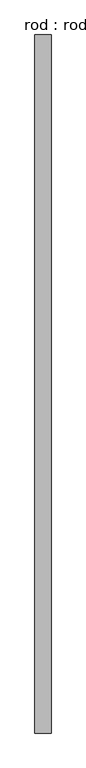
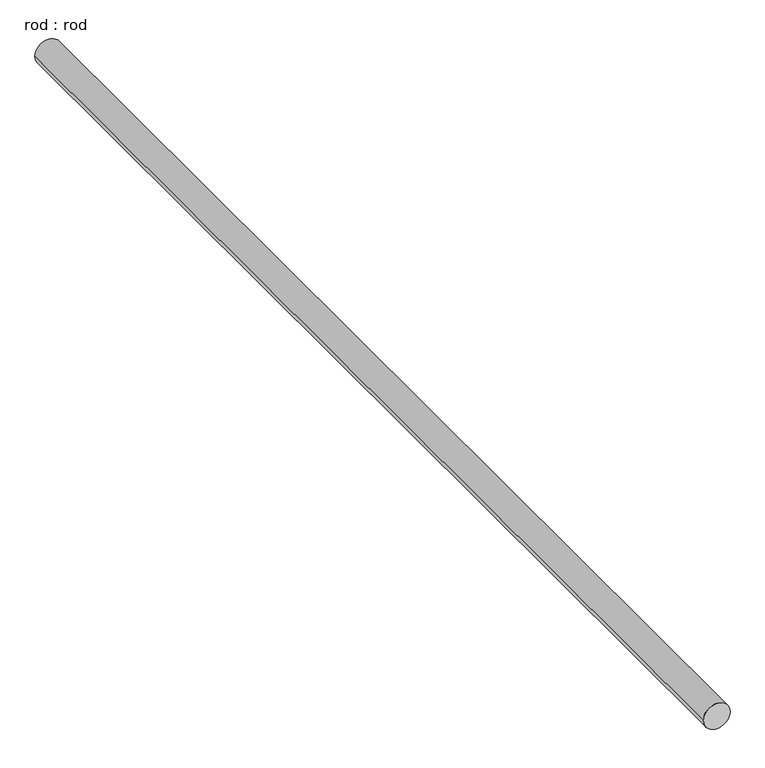
"""IFC4 building model written with IfcOpenShell, lengths in millimetres: proxy geometry, rod : rod."""

import ifcopenshell
import ifcopenshell.guid

model = None  # the IFC model being written
_history = None  # IfcOwnerHistory: only IFC2X3 demands one
_inside = {}  # id of a spatial element -> (the spatial element, [elements in it])
_under = {}  # id of a project, library or spatial element -> (it, [spatial elements below it])
_declared = {}  # id of a project -> (the project, [libraries it declares])
_typed = {}  # id of a type object -> (the type object, [elements of that type])
_made_of = {}  # id of a material, layer set ... -> (it, [elements and type objects made of it])


def new_model(schema):
    """Start an empty IFC model of exactly this schema.

    Asked for "IFC4X3", IfcOpenShell would pick the latest addendum, in which some entities
    have other attributes; the version numbers below select the first issue.
    IFC2X3 requires an IfcOwnerHistory on every rooted entity: one is made here for all.
    """
    global model, _history
    if schema == "IFC4X3":
        model = ifcopenshell.file(schema_version=(4, 3, 0, 0))
    else:
        model = ifcopenshell.file(schema=schema)
    _inside.clear()
    _under.clear()
    _declared.clear()
    _typed.clear()
    _made_of.clear()
    _history = None
    if model.schema == "IFC2X3":
        org = make("IfcOrganization", Name="unknown")
        user = make(
            "IfcPersonAndOrganization",
            ThePerson=make("IfcPerson", FamilyName="unknown"),
            TheOrganization=org,
        )
        app = make(
            "IfcApplication",
            ApplicationDeveloper=org,
            Version="unknown",
            ApplicationFullName="unknown",
            ApplicationIdentifier="unknown",
        )
        _history = make(
            "IfcOwnerHistory",
            OwningUser=user,
            OwningApplication=app,
            ChangeAction="ADDED",
            CreationDate=0,
        )
    return model


def make(cls, **values):
    """One entity of the class cls with the attributes given. An attribute that is None is left unset."""
    return model.create_entity(
        cls, **{name: value for name, value in values.items() if value is not None}
    )


def rooted(cls, **values):
    """An entity with a GlobalId (a new one), such as an element, a storey or a relation."""
    return make(cls, GlobalId=ifcopenshell.guid.new(), OwnerHistory=_history, **values)


def si_unit(unit_type, name, prefix=None):
    """IfcSIUnit, for example si_unit("LENGTHUNIT", "METRE", prefix="MILLI")."""
    return make("IfcSIUnit", UnitType=unit_type, Prefix=prefix, Name=name)


def assignment(units):
    """IfcUnitAssignment: the units of a project."""
    return None if units is None else make("IfcUnitAssignment", Units=units)


def point(xyz):
    """IfcCartesianPoint."""
    return None if xyz is None else make("IfcCartesianPoint", Coordinates=xyz)


def direction(xyz):
    """IfcDirection."""
    return None if xyz is None else make("IfcDirection", DirectionRatios=xyz)


def frame(location, z_axis=None, x_axis=None):
    """IfcAxis2Placement3D, a coordinate frame: its origin and axes. An axis left out is left unset."""
    return make(
        "IfcAxis2Placement3D",
        Location=point(location),
        Axis=direction(z_axis),
        RefDirection=direction(x_axis),
    )


def frame_2d(location, x_axis=None):
    """IfcAxis2Placement2D, a coordinate frame in the plane: its origin and x axis."""
    return make(
        "IfcAxis2Placement2D", Location=point(location), RefDirection=direction(x_axis)
    )


def origin():
    """The frame at (0, 0, 0) with its axes left unset."""
    return frame((0.0, 0.0, 0.0))


def place(relative_to, where):
    """IfcLocalPlacement: puts the frame where relative to a parent placement (None: the world)."""
    return make(
        "IfcLocalPlacement", PlacementRelTo=relative_to, RelativePlacement=where
    )


def context(
    kind, dimensions, precision=None, world=None, true_north=None, identifier=None
):
    """IfcGeometricRepresentationContext, for example the 3D "Model" context."""
    return make(
        "IfcGeometricRepresentationContext",
        ContextIdentifier=identifier,
        ContextType=kind,
        CoordinateSpaceDimension=dimensions,
        Precision=precision,
        WorldCoordinateSystem=world,
        TrueNorth=true_north,
    )


def project(units=None, contexts=None):
    """IfcProject with its units and contexts."""
    return rooted(
        "IfcProject",
        Name="project",
        RepresentationContexts=contexts,
        UnitsInContext=assignment(units),
    )


def spatial(cls, under=None, at=None, **own):
    """A site, building, storey or space (cls), placed at a placement, below another one or the project."""
    s = rooted(cls, ObjectPlacement=at, **own)
    if under is not None:
        _under.setdefault(under.id(), (under, []))[1].append(s)
    return s


def circle_curve(where, radius):
    """IfcCircle in the frame where."""
    return make("IfcCircle", Position=where, Radius=radius)


def trimmed(basis, trim1, trim2, sense, master):
    """IfcTrimmedCurve: the piece of a basis curve between two trims."""
    return make(
        "IfcTrimmedCurve",
        BasisCurve=basis,
        Trim1=trim1,
        Trim2=trim2,
        SenseAgreement=sense,
        MasterRepresentation=master,
    )


def segment(curve, same_sense, transition):
    """IfcCompositeCurveSegment."""
    return make(
        "IfcCompositeCurveSegment",
        Transition=transition,
        SameSense=same_sense,
        ParentCurve=curve,
    )


def composite_curve(segments, self_intersect=None):
    """IfcCompositeCurve: segments joined end to end."""
    return make("IfcCompositeCurve", Segments=segments, SelfIntersect=self_intersect)


def outline(outer, holes=None, kind="AREA"):
    """IfcArbitraryClosedProfileDef: a profile drawn as a closed curve; with holes, ...WithVoids."""
    if holes is None:
        return make("IfcArbitraryClosedProfileDef", ProfileType=kind, OuterCurve=outer)
    return make(
        "IfcArbitraryProfileDefWithVoids",
        ProfileType=kind,
        OuterCurve=outer,
        InnerCurves=holes,
    )


def extrude(swept, where, along, depth):
    """IfcExtrudedAreaSolid: the profile swept, set in the frame where, extruded along a direction by depth."""
    return make(
        "IfcExtrudedAreaSolid",
        SweptArea=swept,
        Position=where,
        ExtrudedDirection=direction(along),
        Depth=depth,
    )


def shape(context_of_items, identifier, shape_type, items):
    """IfcShapeRepresentation: the items that make up one representation, for example the "Body"."""
    return make(
        "IfcShapeRepresentation",
        ContextOfItems=context_of_items,
        RepresentationIdentifier=identifier,
        RepresentationType=shape_type,
        Items=items,
    )


def source(mapping_origin, context_of_items, identifier, shape_type, items):
    """IfcRepresentationMap: a shape defined once, which mapped items show again and again."""
    return make(
        "IfcRepresentationMap",
        MappingOrigin=mapping_origin,
        MappedRepresentation=shape(context_of_items, identifier, shape_type, items),
    )


def transform(
    local_origin,
    x_axis=None,
    y_axis=None,
    z_axis=None,
    scale=None,
    scale2=None,
    scale3=None,
    uniform=True,
):
    """IfcCartesianTransformationOperator3D, or its non-uniform kind. x_axis, y_axis, z_axis: its Axis1, 2, 3."""
    if uniform:
        return make(
            "IfcCartesianTransformationOperator3D",
            Axis1=direction(x_axis),
            Axis2=direction(y_axis),
            LocalOrigin=point(local_origin),
            Scale=scale,
            Axis3=direction(z_axis),
        )
    return make(
        "IfcCartesianTransformationOperator3DnonUniform",
        Axis1=direction(x_axis),
        Axis2=direction(y_axis),
        LocalOrigin=point(local_origin),
        Scale=scale,
        Axis3=direction(z_axis),
        Scale2=scale2,
        Scale3=scale3,
    )


def mapped(mapping_source, mapping_target):
    """IfcMappedItem: shows the shape of a source again, moved by a transform."""
    return make(
        "IfcMappedItem", MappingSource=mapping_source, MappingTarget=mapping_target
    )


def made_of(thing, what):
    """Note that an element or type object is made of a material, layer set ...; save() writes the relation."""
    if what is not None:
        _made_of.setdefault(what.id(), (what, []))[1].append(thing)
    return thing


def element(
    cls,
    number,
    at=None,
    inside=None,
    cuts=None,
    type_object=None,
    material=None,
    context=None,
    identifier="Body",
    shape_type=None,
    held_by="IfcProductDefinitionShape",
    body=None,
    shapes=None,
    **own,
):
    """One element of the class cls, such as IfcWall. Its Tag is "e" and its number.

    at: its placement. inside: the storey or other place that contains it. cuts: it is an
    opening in that element (IfcRelVoidsElement). A single representation is given by context,
    identifier, shape_type and body (its items); several are given by shapes. held_by: the class
    of the entity that holds the representations. save() writes the other relations.
    """
    e = rooted(cls, Tag="e%d" % number, ObjectPlacement=at, **own)
    if body is not None:
        shapes = [shape(context, identifier, shape_type, body)]
    if shapes is not None:
        e.Representation = make(held_by, Representations=shapes)
    if inside is not None:
        _inside.setdefault(inside.id(), (inside, []))[1].append(e)
    if cuts is not None:
        rooted(
            "IfcRelVoidsElement", RelatingBuildingElement=cuts, RelatedOpeningElement=e
        )
    if type_object is not None:
        _typed.setdefault(type_object.id(), (type_object, []))[1].append(e)
    return made_of(e, material)


def aggregate(whole, parts):
    """IfcRelAggregates: a whole, such as a stair, and the parts it consists of."""
    return rooted("IfcRelAggregates", RelatingObject=whole, RelatedObjects=parts)


def save(model, path):
    """Write the relations noted so far, then the file.

    IfcRelAggregates (storeys below a building ...), IfcRelContainedInSpatialStructure (elements
    in a storey), IfcRelDefinesByType, IfcRelAssociatesMaterial and IfcRelDeclares: one each for
    every whole, place, type object, material and project.
    """
    for whole, parts in _under.values():
        aggregate(whole, parts)
    for where, things in _inside.values():
        rooted(
            "IfcRelContainedInSpatialStructure",
            RelatedElements=things,
            RelatingStructure=where,
        )
    for kind, things in _typed.values():
        rooted("IfcRelDefinesByType", RelatedObjects=things, RelatingType=kind)
    for what, things in _made_of.values():
        rooted("IfcRelAssociatesMaterial", RelatedObjects=things, RelatingMaterial=what)
    for by, libraries in _declared.values():
        rooted("IfcRelDeclares", RelatingContext=by, RelatedDefinitions=libraries)
    model.write(path)


def rod_rod_9104e5f4(model_context):
    return source(origin(), model_context, "Body", "SweptSolid", [
        extrude(outline(composite_curve([segment(trimmed(circle_curve(frame_2d((0.0108462, 0.0)), 200.0), [point((0.0108462, 200.0))], [point((0.0108462, -200.0))], False, "CARTESIAN"), True, "CONTINUOUS"), segment(trimmed(circle_curve(frame_2d((0.0108462, 0.0)), 200.0), [point((0.0108462, -200.0))], [point((0.0108462, 200.0))], False, "CARTESIAN"), True, "CONTINUOUS")], self_intersect=False)), frame((0.0, -4573.9380513, 0.0), z_axis=(0.0, 1.0, 0.0), x_axis=(0.0, 0.0, 1.0)), (0.0, 0.0, 1.0), 17333.3333333),
    ])


if __name__ == "__main__":
    model = new_model("IFC4")
    model_context = context("Model", 3, world=origin())
    ifc_project = project(units=[si_unit("LENGTHUNIT", "METRE", prefix="MILLI")], contexts=[model_context])
    site = spatial("IfcSite", under=ifc_project)
    building = spatial("IfcBuilding", under=site)
    placement = place(None, origin())
    rod_rod_shape = rod_rod_9104e5f4(model_context)
    element("IfcBuildingElementProxy", 1, Name="rod : rod", ObjectType="rod : rod", at=placement, inside=building, context=model_context, shape_type="MappedRepresentation", body=[
        mapped(rod_rod_shape, transform((0.0, 0.0, 0.0), x_axis=(1.0, 0.0, 0.0), y_axis=(0.0, 1.0, 0.0), z_axis=(0.0, 0.0, 1.0))),
    ])
    save(model, "model.ifc")

# Revit data of these elements
# Type "rod : rod"
#   Default Elevation = 0
